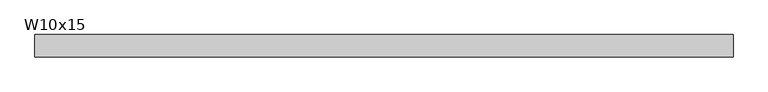
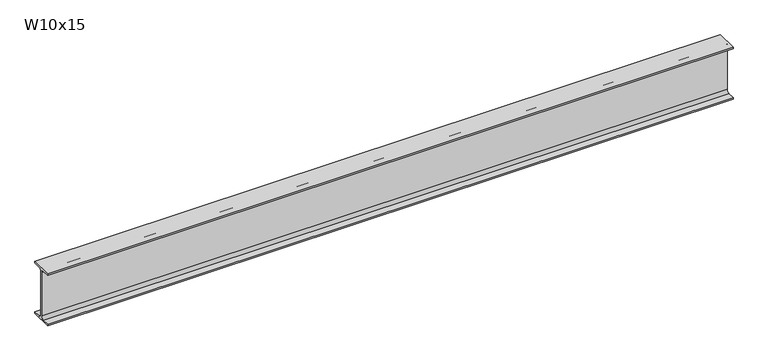
"""IFC4 building model written with IfcOpenShell, lengths in millimetres: beam geometry, RME W-Wide Flange : W10x15."""

from ifc_helpers import new_model, si_unit, point, frame, frame_2d, origin, place, context, project, spatial, polyline, circle_curve, trimmed, segment, composite_curve, outline, extrude, source, transform, mapped, element, save


def w10x15_68d9fed2(model_context):
    return source(origin(), model_context, "Body", "SweptSolid", [
        extrude(outline(composite_curve([segment(polyline([(50.8, -120.142), (50.8, -127.0), (-50.8, -127.0), (-50.8, -120.142), (-16.7005, -120.142)]), True, "CONTINUOUS"), segment(trimmed(circle_curve(frame_2d((-16.7005, -106.3625)), 13.7795), [point((-16.7005, -120.142))], [point((-2.921, -106.3625))], True, "CARTESIAN"), True, "CONTINUOUS"), segment(polyline([(-2.921, -106.3625), (-2.921, 106.3625)]), True, "CONTINUOUS"), segment(trimmed(circle_curve(frame_2d((-16.7005, 106.3625)), 13.7795), [point((-2.921, 106.3625))], [point((-16.7005, 120.142))], True, "CARTESIAN"), True, "CONTINUOUS"), segment(polyline([(-16.7005, 120.142), (-50.8, 120.142), (-50.8, 127.0), (50.8, 127.0), (50.8, 120.142), (16.7005, 120.142)]), True, "CONTINUOUS"), segment(trimmed(circle_curve(frame_2d((16.7005, 106.3625)), 13.7795), [point((16.7005, 120.142))], [point((2.921, 106.3625))], True, "CARTESIAN"), True, "CONTINUOUS"), segment(polyline([(2.921, 106.3625), (2.921, -106.3625)]), True, "CONTINUOUS"), segment(trimmed(circle_curve(frame_2d((16.7005, -106.3625)), 13.7795), [point((2.921, -106.3625))], [point((16.7005, -120.142))], True, "CARTESIAN"), True, "CONTINUOUS"), segment(polyline([(16.7005, -120.142), (50.8, -120.142)]), True, "CONTINUOUS")], self_intersect=False)), frame((-1593.146405, 0.0, 0.0), z_axis=(1.0, 0.0, 0.0), x_axis=(0.0, 1.0, 0.0)), (0.0, 0.0, 1.0), 3184.259384),
    ])


if __name__ == "__main__":
    model = new_model("IFC4")
    model_context = context("Model", 3, world=origin())
    ifc_project = project(units=[si_unit("LENGTHUNIT", "METRE", prefix="MILLI")], contexts=[model_context])
    site = spatial("IfcSite", under=ifc_project)
    building = spatial("IfcBuilding", under=site)
    placement = place(None, origin())
    w10x15_shape = w10x15_68d9fed2(model_context)
    element("IfcBeam", 1, ObjectType="RME W-Wide Flange : W10x15", at=placement, inside=building, context=model_context, shape_type="MappedRepresentation", body=[
        mapped(w10x15_shape, transform((0.0, 0.0, 0.0), x_axis=(1.0, 0.0, 0.0), y_axis=(0.0, 1.0, 0.0), z_axis=(0.0, 0.0, 1.0))),
    ])
    save(model, "model.ifc")

# Revit data of these elements
# Type "RME W-Wide Flange : W10x15"
#   WELD P [instance default] = ""
#   WELD LE [instance default] = ""
#   WELD D [instance default] = ""
#   TOP SECTION SIZE [instance default] = ""
#   TOP SECTION LENGTH [instance default] = ""
#   REMARKS [instance default] = ""
#   REINF TYPE [instance default] = ""
#   Nominal Size = "W24"
#   End Bearing Capacity [instance default] = ""
#   BOT SECTION SIZE [instance default] = ""
#   BOT SECTION LENGTH [instance default] = ""
#   Assembly Code = "B10"
#   W = 15
#   Start Extension Calculation [instance default] = 10' - 0"
#   Start Extension [instance default] = -0' - 0 1/2"
#   End Extension Calculation [instance default] = 10' - 0"
#   End Extension [instance default] = -0' - 0 1/2"
#   Length [instance default] = 5' - 0"
#   bf = 0' - 4"
#   d = 0' - 10"
#   k = 0' - 0 13/16"
#   k2 = 0' - 0.5425"
#   tf = 0' - 0.27"
#   tw = 0' - 0.23"
#   A = 0.030625 SF
#   Structural Material [instance default] = Metal - Steel - ASTM A992
# Element 1 (IfcBeam, "RME W-Wide Flange : W10x15")
#   Length = 9' - 11.03177"
#   Materials on its faces: "Metal - Steel - ASTM A992"
# Materials
#   "Metal - Steel - ASTM A992": class "Metal", colour RGB 255 128 0, transparency 0
